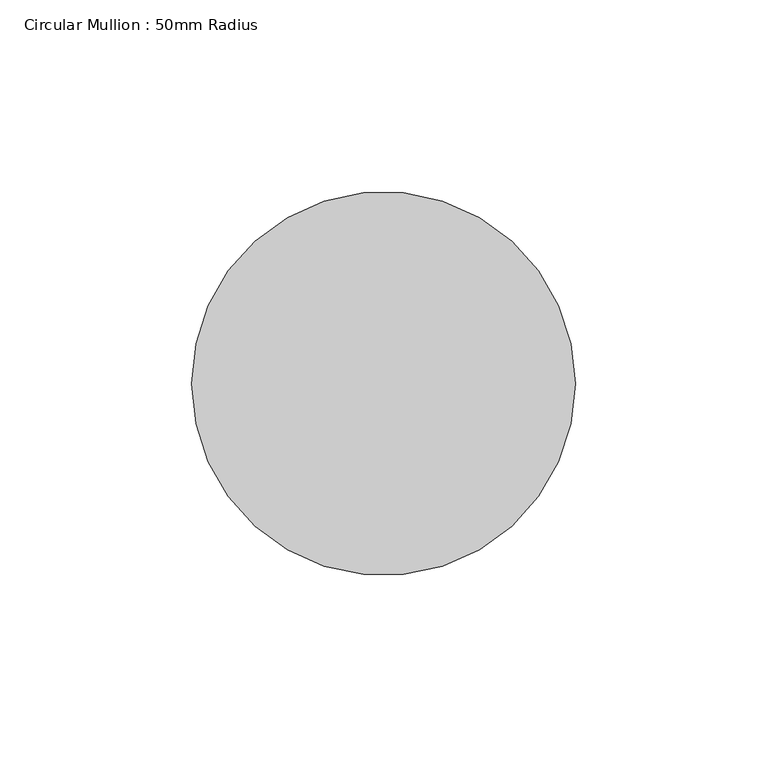
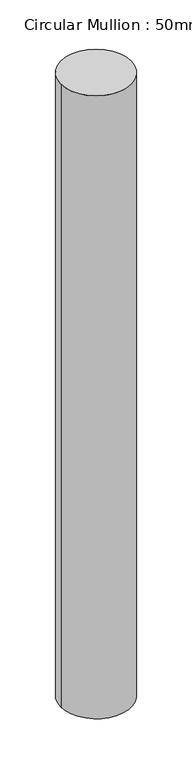
"""IFC4 building model written with IfcOpenShell, lengths in millimetres: member geometry, Circular Mullion : 50mm Radius."""

from ifc_helpers import new_model, si_unit, point, frame, origin, origin_2d, place, context, project, spatial, circle_curve, trimmed, segment, composite_curve, outline, extrude, source, transform, mapped, element, save


def circular_mullion_50mm_radius_d8ddd876(model_context):
    return source(origin(), model_context, "Body", "SweptSolid", [
        extrude(outline(composite_curve([segment(trimmed(circle_curve(origin_2d(), 50.0), [point((50.0, 0.0))], [point((-50.0, 0.0))], False, "CARTESIAN"), True, "CONTINUOUS"), segment(trimmed(circle_curve(origin_2d(), 50.0), [point((-50.0, 0.0))], [point((50.0, 0.0))], False, "CARTESIAN"), True, "CONTINUOUS")], self_intersect=False)), frame((0.0, 0.0, -934.8303218), z_axis=(0.0, 0.0, 1.0), x_axis=(1.0, 0.0, 0.0)), (0.0, 0.0, 1.0), 934.8303218),
    ])


if __name__ == "__main__":
    model = new_model("IFC4")
    model_context = context("Model", 3, world=origin())
    ifc_project = project(units=[si_unit("LENGTHUNIT", "METRE", prefix="MILLI")], contexts=[model_context])
    site = spatial("IfcSite", under=ifc_project)
    building = spatial("IfcBuilding", under=site)
    placement = place(None, origin())
    circular_mullion_50mm_radius_shape = circular_mullion_50mm_radius_d8ddd876(model_context)
    element("IfcMember", 1, ObjectType="Circular Mullion : 50mm Radius", at=placement, inside=building, context=model_context, shape_type="MappedRepresentation", body=[
        mapped(circular_mullion_50mm_radius_shape, transform((0.0, 0.0, 0.0), x_axis=(1.0, 0.0, 0.0), y_axis=(0.0, 1.0, 0.0), z_axis=(0.0, 0.0, 1.0))),
    ])
    save(model, "model.ifc")

# Revit data of these elements
# Type "Circular Mullion : 50mm Radius"
#   built-in parameter 1007350 = 0.164042 (stored number, unit not read)
# Element 1 (IfcMember, "Circular Mullion : 50mm Radius")
#   Materials on its faces: "Aluminium"
# Materials
#   "Aluminium": class "Metal", colour RGB 247 247 247, transparency 0, Description = "Aluminium 6061", Cost = 0
